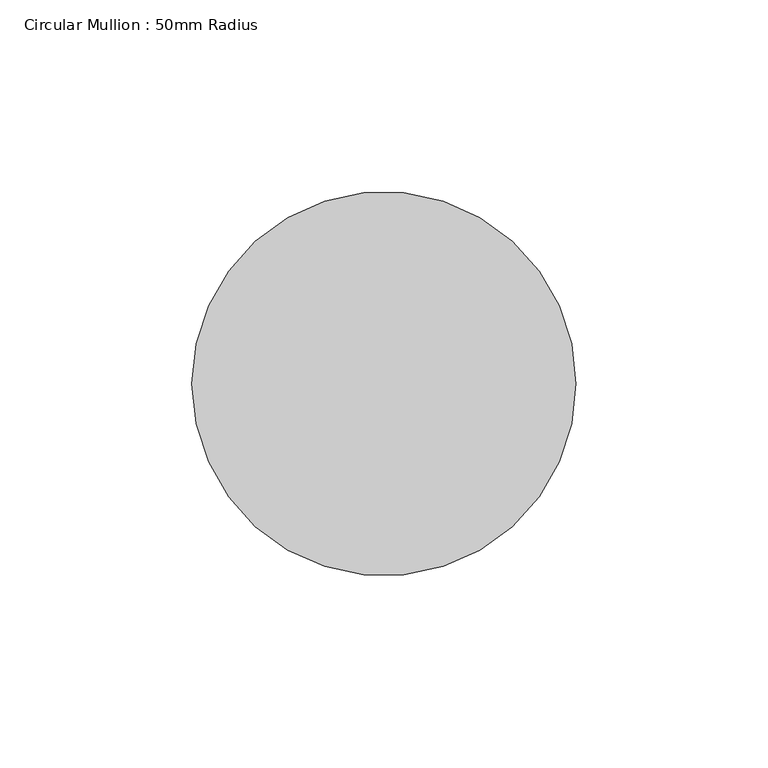
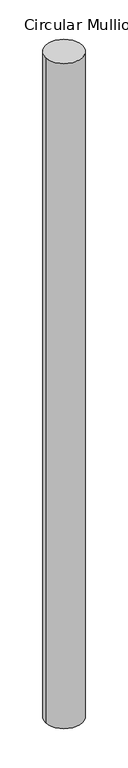
"""IFC4 building model written with IfcOpenShell, lengths in millimetres: member geometry, Circular Mullion : 50mm Radius."""

import ifcopenshell
import ifcopenshell.guid

model = None  # the IFC model being written
_history = None  # IfcOwnerHistory: only IFC2X3 demands one
_inside = {}  # id of a spatial element -> (the spatial element, [elements in it])
_under = {}  # id of a project, library or spatial element -> (it, [spatial elements below it])
_declared = {}  # id of a project -> (the project, [libraries it declares])
_typed = {}  # id of a type object -> (the type object, [elements of that type])
_made_of = {}  # id of a material, layer set ... -> (it, [elements and type objects made of it])


def new_model(schema):
    """Start an empty IFC model of exactly this schema.

    Asked for "IFC4X3", IfcOpenShell would pick the latest addendum, in which some entities
    have other attributes; the version numbers below select the first issue.
    IFC2X3 requires an IfcOwnerHistory on every rooted entity: one is made here for all.
    """
    global model, _history
    if schema == "IFC4X3":
        model = ifcopenshell.file(schema_version=(4, 3, 0, 0))
    else:
        model = ifcopenshell.file(schema=schema)
    _inside.clear()
    _under.clear()
    _declared.clear()
    _typed.clear()
    _made_of.clear()
    _history = None
    if model.schema == "IFC2X3":
        org = make("IfcOrganization", Name="unknown")
        user = make(
            "IfcPersonAndOrganization",
            ThePerson=make("IfcPerson", FamilyName="unknown"),
            TheOrganization=org,
        )
        app = make(
            "IfcApplication",
            ApplicationDeveloper=org,
            Version="unknown",
            ApplicationFullName="unknown",
            ApplicationIdentifier="unknown",
        )
        _history = make(
            "IfcOwnerHistory",
            OwningUser=user,
            OwningApplication=app,
            ChangeAction="ADDED",
            CreationDate=0,
        )
    return model


def make(cls, **values):
    """One entity of the class cls with the attributes given. An attribute that is None is left unset."""
    return model.create_entity(
        cls, **{name: value for name, value in values.items() if value is not None}
    )


def rooted(cls, **values):
    """An entity with a GlobalId (a new one), such as an element, a storey or a relation."""
    return make(cls, GlobalId=ifcopenshell.guid.new(), OwnerHistory=_history, **values)


def si_unit(unit_type, name, prefix=None):
    """IfcSIUnit, for example si_unit("LENGTHUNIT", "METRE", prefix="MILLI")."""
    return make("IfcSIUnit", UnitType=unit_type, Prefix=prefix, Name=name)


def assignment(units):
    """IfcUnitAssignment: the units of a project."""
    return None if units is None else make("IfcUnitAssignment", Units=units)


def point(xyz):
    """IfcCartesianPoint."""
    return None if xyz is None else make("IfcCartesianPoint", Coordinates=xyz)


def direction(xyz):
    """IfcDirection."""
    return None if xyz is None else make("IfcDirection", DirectionRatios=xyz)


def frame(location, z_axis=None, x_axis=None):
    """IfcAxis2Placement3D, a coordinate frame: its origin and axes. An axis left out is left unset."""
    return make(
        "IfcAxis2Placement3D",
        Location=point(location),
        Axis=direction(z_axis),
        RefDirection=direction(x_axis),
    )


def frame_2d(location, x_axis=None):
    """IfcAxis2Placement2D, a coordinate frame in the plane: its origin and x axis."""
    return make(
        "IfcAxis2Placement2D", Location=point(location), RefDirection=direction(x_axis)
    )


def origin():
    """The frame at (0, 0, 0) with its axes left unset."""
    return frame((0.0, 0.0, 0.0))


def place(relative_to, where):
    """IfcLocalPlacement: puts the frame where relative to a parent placement (None: the world)."""
    return make(
        "IfcLocalPlacement", PlacementRelTo=relative_to, RelativePlacement=where
    )


def context(
    kind, dimensions, precision=None, world=None, true_north=None, identifier=None
):
    """IfcGeometricRepresentationContext, for example the 3D "Model" context."""
    return make(
        "IfcGeometricRepresentationContext",
        ContextIdentifier=identifier,
        ContextType=kind,
        CoordinateSpaceDimension=dimensions,
        Precision=precision,
        WorldCoordinateSystem=world,
        TrueNorth=true_north,
    )


def project(units=None, contexts=None):
    """IfcProject with its units and contexts."""
    return rooted(
        "IfcProject",
        Name="project",
        RepresentationContexts=contexts,
        UnitsInContext=assignment(units),
    )


def spatial(cls, under=None, at=None, **own):
    """A site, building, storey or space (cls), placed at a placement, below another one or the project."""
    s = rooted(cls, ObjectPlacement=at, **own)
    if under is not None:
        _under.setdefault(under.id(), (under, []))[1].append(s)
    return s


def circle_curve(where, radius):
    """IfcCircle in the frame where."""
    return make("IfcCircle", Position=where, Radius=radius)


def trimmed(basis, trim1, trim2, sense, master):
    """IfcTrimmedCurve: the piece of a basis curve between two trims."""
    return make(
        "IfcTrimmedCurve",
        BasisCurve=basis,
        Trim1=trim1,
        Trim2=trim2,
        SenseAgreement=sense,
        MasterRepresentation=master,
    )


def segment(curve, same_sense, transition):
    """IfcCompositeCurveSegment."""
    return make(
        "IfcCompositeCurveSegment",
        Transition=transition,
        SameSense=same_sense,
        ParentCurve=curve,
    )


def composite_curve(segments, self_intersect=None):
    """IfcCompositeCurve: segments joined end to end."""
    return make("IfcCompositeCurve", Segments=segments, SelfIntersect=self_intersect)


def outline(outer, holes=None, kind="AREA"):
    """IfcArbitraryClosedProfileDef: a profile drawn as a closed curve; with holes, ...WithVoids."""
    if holes is None:
        return make("IfcArbitraryClosedProfileDef", ProfileType=kind, OuterCurve=outer)
    return make(
        "IfcArbitraryProfileDefWithVoids",
        ProfileType=kind,
        OuterCurve=outer,
        InnerCurves=holes,
    )


def extrude(swept, where, along, depth):
    """IfcExtrudedAreaSolid: the profile swept, set in the frame where, extruded along a direction by depth."""
    return make(
        "IfcExtrudedAreaSolid",
        SweptArea=swept,
        Position=where,
        ExtrudedDirection=direction(along),
        Depth=depth,
    )


def shape(context_of_items, identifier, shape_type, items):
    """IfcShapeRepresentation: the items that make up one representation, for example the "Body"."""
    return make(
        "IfcShapeRepresentation",
        ContextOfItems=context_of_items,
        RepresentationIdentifier=identifier,
        RepresentationType=shape_type,
        Items=items,
    )


def source(mapping_origin, context_of_items, identifier, shape_type, items):
    """IfcRepresentationMap: a shape defined once, which mapped items show again and again."""
    return make(
        "IfcRepresentationMap",
        MappingOrigin=mapping_origin,
        MappedRepresentation=shape(context_of_items, identifier, shape_type, items),
    )


def transform(
    local_origin,
    x_axis=None,
    y_axis=None,
    z_axis=None,
    scale=None,
    scale2=None,
    scale3=None,
    uniform=True,
):
    """IfcCartesianTransformationOperator3D, or its non-uniform kind. x_axis, y_axis, z_axis: its Axis1, 2, 3."""
    if uniform:
        return make(
            "IfcCartesianTransformationOperator3D",
            Axis1=direction(x_axis),
            Axis2=direction(y_axis),
            LocalOrigin=point(local_origin),
            Scale=scale,
            Axis3=direction(z_axis),
        )
    return make(
        "IfcCartesianTransformationOperator3DnonUniform",
        Axis1=direction(x_axis),
        Axis2=direction(y_axis),
        LocalOrigin=point(local_origin),
        Scale=scale,
        Axis3=direction(z_axis),
        Scale2=scale2,
        Scale3=scale3,
    )


def mapped(mapping_source, mapping_target):
    """IfcMappedItem: shows the shape of a source again, moved by a transform."""
    return make(
        "IfcMappedItem", MappingSource=mapping_source, MappingTarget=mapping_target
    )


def made_of(thing, what):
    """Note that an element or type object is made of a material, layer set ...; save() writes the relation."""
    if what is not None:
        _made_of.setdefault(what.id(), (what, []))[1].append(thing)
    return thing


def element(
    cls,
    number,
    at=None,
    inside=None,
    cuts=None,
    type_object=None,
    material=None,
    context=None,
    identifier="Body",
    shape_type=None,
    held_by="IfcProductDefinitionShape",
    body=None,
    shapes=None,
    **own,
):
    """One element of the class cls, such as IfcWall. Its Tag is "e" and its number.

    at: its placement. inside: the storey or other place that contains it. cuts: it is an
    opening in that element (IfcRelVoidsElement). A single representation is given by context,
    identifier, shape_type and body (its items); several are given by shapes. held_by: the class
    of the entity that holds the representations. save() writes the other relations.
    """
    e = rooted(cls, Tag="e%d" % number, ObjectPlacement=at, **own)
    if body is not None:
        shapes = [shape(context, identifier, shape_type, body)]
    if shapes is not None:
        e.Representation = make(held_by, Representations=shapes)
    if inside is not None:
        _inside.setdefault(inside.id(), (inside, []))[1].append(e)
    if cuts is not None:
        rooted(
            "IfcRelVoidsElement", RelatingBuildingElement=cuts, RelatedOpeningElement=e
        )
    if type_object is not None:
        _typed.setdefault(type_object.id(), (type_object, []))[1].append(e)
    return made_of(e, material)


def aggregate(whole, parts):
    """IfcRelAggregates: a whole, such as a stair, and the parts it consists of."""
    return rooted("IfcRelAggregates", RelatingObject=whole, RelatedObjects=parts)


def save(model, path):
    """Write the relations noted so far, then the file.

    IfcRelAggregates (storeys below a building ...), IfcRelContainedInSpatialStructure (elements
    in a storey), IfcRelDefinesByType, IfcRelAssociatesMaterial and IfcRelDeclares: one each for
    every whole, place, type object, material and project.
    """
    for whole, parts in _under.values():
        aggregate(whole, parts)
    for where, things in _inside.values():
        rooted(
            "IfcRelContainedInSpatialStructure",
            RelatedElements=things,
            RelatingStructure=where,
        )
    for kind, things in _typed.values():
        rooted("IfcRelDefinesByType", RelatedObjects=things, RelatingType=kind)
    for what, things in _made_of.values():
        rooted("IfcRelAssociatesMaterial", RelatedObjects=things, RelatingMaterial=what)
    for by, libraries in _declared.values():
        rooted("IfcRelDeclares", RelatingContext=by, RelatedDefinitions=libraries)
    model.write(path)


def circular_mullion_50mm_radius_9376a9a5(model_context):
    return source(origin(), model_context, "Body", "SweptSolid", [
        extrude(outline(composite_curve([segment(trimmed(circle_curve(frame_2d((-50.0, 0.0)), 50.0), [point((0.0, 0.0))], [point((-100.0, 0.0))], False, "CARTESIAN"), True, "CONTINUOUS"), segment(trimmed(circle_curve(frame_2d((-50.0, 0.0)), 50.0), [point((-100.0, 0.0))], [point((0.0, 0.0))], False, "CARTESIAN"), True, "CONTINUOUS")], self_intersect=False)), frame((0.0, 0.0, -1911.5310404), z_axis=(0.0, 0.0, 1.0), x_axis=(1.0, 0.0, 0.0)), (0.0, 0.0, 1.0), 1911.5310404),
    ])


if __name__ == "__main__":
    model = new_model("IFC4")
    model_context = context("Model", 3, world=origin())
    ifc_project = project(units=[si_unit("LENGTHUNIT", "METRE", prefix="MILLI")], contexts=[model_context])
    site = spatial("IfcSite", under=ifc_project)
    building = spatial("IfcBuilding", under=site)
    placement = place(None, origin())
    circular_mullion_50mm_radius_shape = circular_mullion_50mm_radius_9376a9a5(model_context)
    element("IfcMember", 1, ObjectType="Circular Mullion : 50mm Radius", at=placement, inside=building, context=model_context, shape_type="MappedRepresentation", body=[
        mapped(circular_mullion_50mm_radius_shape, transform((0.0, 0.0, 0.0), x_axis=(1.0, 0.0, 0.0), y_axis=(0.0, 1.0, 0.0), z_axis=(0.0, 0.0, 1.0))),
    ])
    save(model, "model.ifc")

# Revit data of these elements
# Type "Circular Mullion : 50mm Radius"
#   built-in parameter 1007350 = 0.164042 (stored number, unit not read)
# Element 1 (IfcMember, "Circular Mullion : 50mm Radius")
#   Materials on its faces: "Aluminium"
# Materials
#   "Aluminium": class "Metal", colour RGB 247 247 247, transparency 0, Description = "Aluminium 6061", Cost = 0
